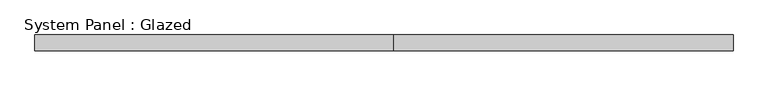
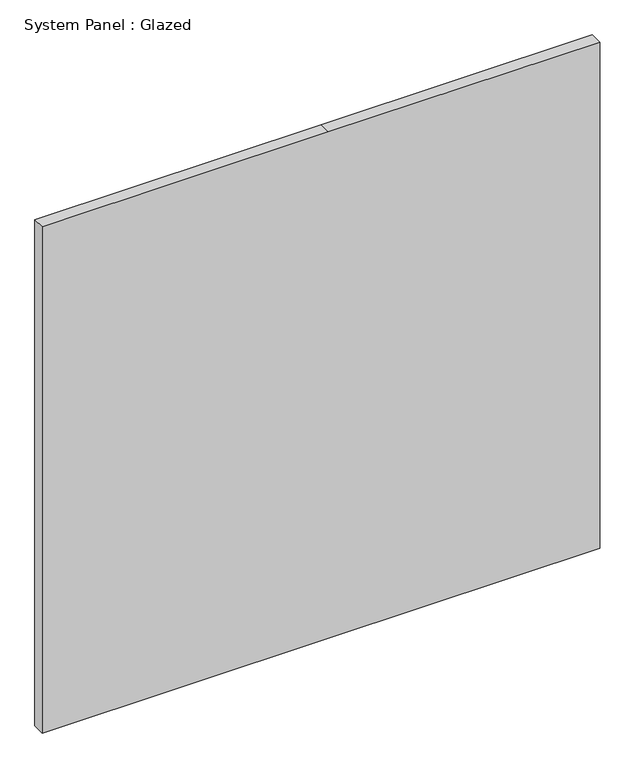
"""IFC4 building model written with IfcOpenShell, lengths in millimetres: plate geometry, System Panel : Glazed."""

from ifc_helpers import new_model, si_unit, frame, origin, place, context, project, spatial, polyline, outline, extrude, source, transform, mapped, element, save


def system_panel_glazed_fceb0f72(model_context):
    return source(origin(), model_context, "Body", "SweptSolid", [
        extrude(outline(polyline([(0.0, -1119.5), (0.0, 30.5), (0.0, 1119.5), (2150.0, 1119.5), (2150.0, 30.5), (2150.0, -1119.5), (0.0, -1119.5)])), frame((0.0, -25.0, 0.0), z_axis=(0.0, 1.0, 0.0), x_axis=(0.0, 0.0, 1.0)), (0.0, 0.0, 1.0), 50.0),
    ])


if __name__ == "__main__":
    model = new_model("IFC4")
    model_context = context("Model", 3, world=origin())
    ifc_project = project(units=[si_unit("LENGTHUNIT", "METRE", prefix="MILLI")], contexts=[model_context])
    site = spatial("IfcSite", under=ifc_project)
    building = spatial("IfcBuilding", under=site)
    placement = place(None, origin())
    system_panel_glazed_shape = system_panel_glazed_fceb0f72(model_context)
    element("IfcPlate", 1, ObjectType="System Panel : Glazed", at=placement, inside=building, context=model_context, shape_type="MappedRepresentation", body=[
        mapped(system_panel_glazed_shape, transform((0.0, 0.0, 0.0), x_axis=(1.0, 0.0, 0.0), y_axis=(0.0, 1.0, 0.0), z_axis=(0.0, 0.0, 1.0))),
    ])
    save(model, "model.ifc")

# Revit data of these elements
# Type "System Panel : Glazed"
#   Type Mark = "CW-GLASS"
# Element 1 (IfcPlate, "System Panel : Glazed")
#   Materials on its faces: "Glass_Clear"
# Materials
#   "Glass_Clear": class "Glass", colour RGB 128 128 255, transparency 0.8, Comments = "Rendering appearance not upgraded ", Cost = 0
